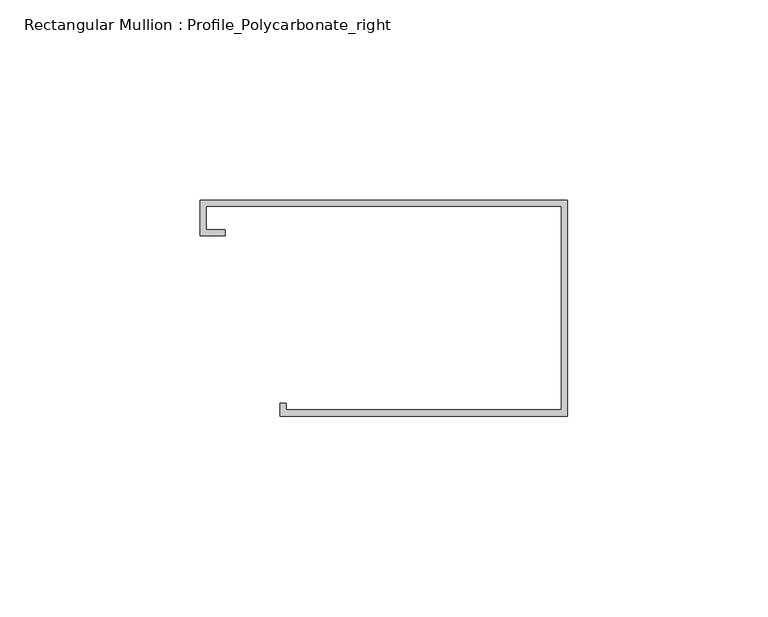
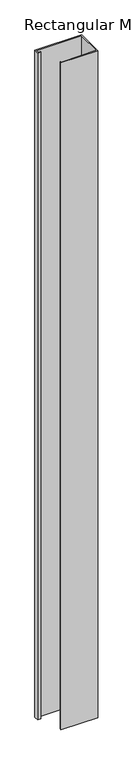
"""IFC4 building model written with IfcOpenShell, lengths in millimetres: member geometry, Rectangular Mullion : Profile_Polycarbonate_right."""

from ifc_helpers import new_model, si_unit, frame, origin, place, context, project, spatial, polyline, outline, extrude, source, transform, mapped, element, save


def rectangular_mullion_profile_polycarbonate_right_90581fae(model_context):
    return source(origin(), model_context, "Body", "SweptSolid", [
        extrude(outline(polyline([(0.0, 28.984575), (0.0, -25.015825), (-71.9836, -25.015825), (-71.9836, -21.840825), (-70.3961, -21.840825), (-70.3961, -23.428325), (-1.5875, -23.428325), (-1.5875, 27.397075), (-90.4113, 27.397075), (-90.4113, 21.580475), (-85.6488, 21.580475), (-85.6488, 19.992975), (-91.9988, 19.992975), (-91.9988, 28.984575), (0.0, 28.984575)])), frame((0.0, 0.0, -1384.6898973), z_axis=(0.0, 0.0, 1.0), x_axis=(1.0, 0.0, 0.0)), (0.0, 0.0, 1.0), 1384.6898973),
    ])


if __name__ == "__main__":
    model = new_model("IFC4")
    model_context = context("Model", 3, world=origin())
    ifc_project = project(units=[si_unit("LENGTHUNIT", "METRE", prefix="MILLI")], contexts=[model_context])
    site = spatial("IfcSite", under=ifc_project)
    building = spatial("IfcBuilding", under=site)
    placement = place(None, origin())
    rectangular_mullion_profile_polycarbonate_right_shape = rectangular_mullion_profile_polycarbonate_right_90581fae(model_context)
    element("IfcMember", 1, ObjectType="Rectangular Mullion : Profile_Polycarbonate_right", at=placement, inside=building, context=model_context, shape_type="MappedRepresentation", body=[
        mapped(rectangular_mullion_profile_polycarbonate_right_shape, transform((0.0, 0.0, 0.0), x_axis=(1.0, 0.0, 0.0), y_axis=(0.0, 1.0, 0.0), z_axis=(0.0, 0.0, 1.0))),
    ])
    save(model, "model.ifc")

# Revit data of these elements
# Type "Rectangular Mullion : Profile_Polycarbonate_right"
#   built-in parameter 1007322 = 0.177167 (stored number, unit not read)
#   built-in parameter 1007321 = 0 (stored number, unit not read)
#   built-in parameter 1007320 = 0.00520833 (stored number, unit not read)
